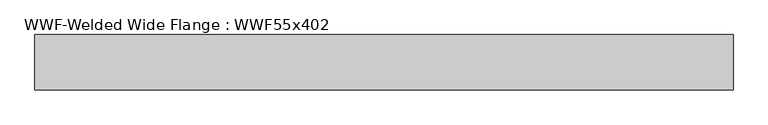
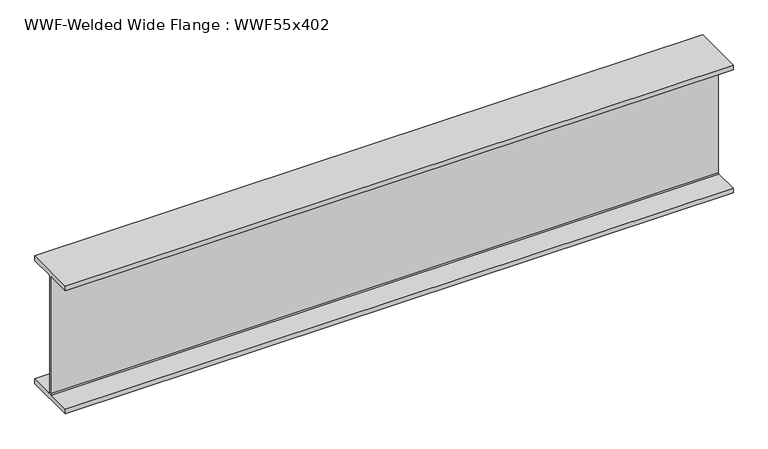
"""IFC4 building model written with IfcOpenShell, lengths in millimetres: beam geometry, WWF-Welded Wide Flange : WWF55x402."""

from ifc_helpers import new_model, si_unit, frame, origin, place, context, project, spatial, polyline, outline, extrude, source, transform, mapped, element, save


def wwf_welded_wide_flange_wwf55x402_d46538ab(model_context):
    return source(origin(), model_context, "Body", "SweptSolid", [
        extrude(outline(polyline([(274.955, -649.986), (274.955, -700.024), (-274.955, -700.024), (-274.955, -649.986), (-19.05, -649.986), (-8.001, -638.937), (-8.001, 638.937), (-19.05, 649.986), (-274.955, 649.986), (-274.955, 700.024), (274.955, 700.024), (274.955, 649.986), (19.05, 649.986), (8.001, 638.937), (8.001, -638.937), (19.05, -649.986), (274.955, -649.986)])), frame((-3472.22503, 0.0, 0.0), z_axis=(1.0, 0.0, 0.0), x_axis=(0.0, 1.0, 0.0)), (0.0, 0.0, 1.0), 6931.7500593),
    ])


if __name__ == "__main__":
    model = new_model("IFC4")
    model_context = context("Model", 3, world=origin())
    ifc_project = project(units=[si_unit("LENGTHUNIT", "METRE", prefix="MILLI")], contexts=[model_context])
    site = spatial("IfcSite", under=ifc_project)
    building = spatial("IfcBuilding", under=site)
    placement = place(None, origin())
    wwf_welded_wide_flange_wwf55x402_shape = wwf_welded_wide_flange_wwf55x402_d46538ab(model_context)
    element("IfcBeam", 1, ObjectType="WWF-Welded Wide Flange : WWF55x402", at=placement, inside=building, context=model_context, shape_type="MappedRepresentation", body=[
        mapped(wwf_welded_wide_flange_wwf55x402_shape, transform((0.0, 0.0, 0.0), x_axis=(1.0, 0.0, 0.0), y_axis=(0.0, 1.0, 0.0), z_axis=(0.0, 0.0, 1.0))),
    ])
    save(model, "model.ifc")

# Revit data of these elements
# Type "WWF-Welded Wide Flange : WWF55x402"
#   Assembly Code = "B10"
#   Nominal d = "12"
#   W = 402
#   Length [instance default] = 1524 mm
#   bf = 549.91 mm
#   d = 1400.048 mm
#   k = 19.05 mm
#   tf = 50.038 mm
#   tw = 16.002 mm
#   A = 0.0761289 m²
#   Structural Material [instance default] = Steel ASTM A572
# Element 1 (IfcBeam, "WWF-Welded Wide Flange : WWF55x402")
#   Structural Material = Metal - Steel 43-275
#   Materials on its faces: "Metal - Steel 43-275"
# Materials
#   "Steel ASTM A572": class "Metal", colour RGB 247 247 247, transparency 0, Description = "Structural steel, high strength low alloy, ASTM - A572 - 50", Cost = 0
#   "Metal - Steel 43-275": class "Metal", colour RGB 247 247 247, transparency 0, Cost = 0
